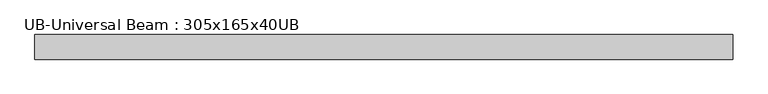
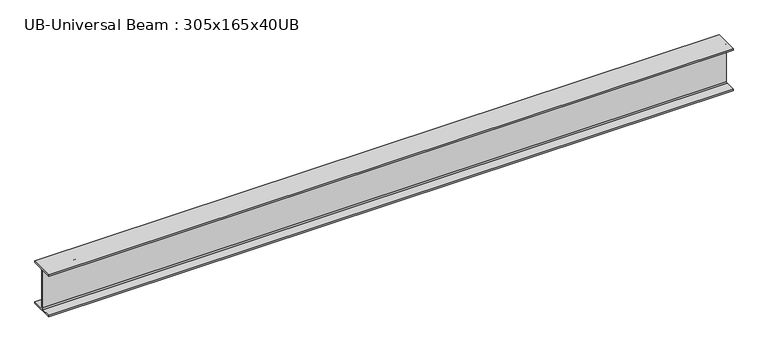
"""IFC4 building model written with IfcOpenShell, lengths in millimetres: beam geometry, UB-Universal Beam : 305x165x40UB."""

from ifc_helpers import new_model, si_unit, point, frame, frame_2d, origin, place, context, project, spatial, polyline, circle_curve, trimmed, segment, composite_curve, outline, extrude, source, transform, mapped, element, save


def ub_universal_beam_305x165x40ub_4e97a9be(model_context):
    return source(origin(), model_context, "Body", "SweptSolid", [
        extrude(outline(composite_curve([segment(polyline([(82.5, -141.5), (82.5, -151.7), (-82.5, -151.7), (-82.5, -141.5), (-11.9, -141.5)]), True, "CONTINUOUS"), segment(trimmed(circle_curve(frame_2d((-11.9, -132.6)), 8.9), [point((-11.9, -141.5))], [point((-3.0, -132.6))], True, "CARTESIAN"), True, "CONTINUOUS"), segment(polyline([(-3.0, -132.6), (-3.0, 132.6)]), True, "CONTINUOUS"), segment(trimmed(circle_curve(frame_2d((-11.9, 132.6)), 8.9), [point((-3.0, 132.6))], [point((-11.9, 141.5))], True, "CARTESIAN"), True, "CONTINUOUS"), segment(polyline([(-11.9, 141.5), (-82.5, 141.5), (-82.5, 151.7), (82.5, 151.7), (82.5, 141.5), (11.9, 141.5)]), True, "CONTINUOUS"), segment(trimmed(circle_curve(frame_2d((11.9, 132.6)), 8.9), [point((11.9, 141.5))], [point((3.0, 132.6))], True, "CARTESIAN"), True, "CONTINUOUS"), segment(polyline([(3.0, 132.6), (3.0, -132.6)]), True, "CONTINUOUS"), segment(trimmed(circle_curve(frame_2d((11.9, -132.6)), 8.9), [point((3.0, -132.6))], [point((11.9, -141.5))], True, "CARTESIAN"), True, "CONTINUOUS"), segment(polyline([(11.9, -141.5), (82.5, -141.5)]), True, "CONTINUOUS")], self_intersect=False)), frame((-2334.65, 0.0, 0.0), z_axis=(1.0, 0.0, 0.0), x_axis=(0.0, 1.0, 0.0)), (0.0, 0.0, 1.0), 4669.3),
    ])


if __name__ == "__main__":
    model = new_model("IFC4")
    model_context = context("Model", 3, world=origin())
    ifc_project = project(units=[si_unit("LENGTHUNIT", "METRE", prefix="MILLI")], contexts=[model_context])
    site = spatial("IfcSite", under=ifc_project)
    building = spatial("IfcBuilding", under=site)
    placement = place(None, origin())
    ub_universal_beam_305x165x40ub_shape = ub_universal_beam_305x165x40ub_4e97a9be(model_context)
    element("IfcBeam", 1, ObjectType="UB-Universal Beam : 305x165x40UB", at=placement, inside=building, context=model_context, shape_type="MappedRepresentation", body=[
        mapped(ub_universal_beam_305x165x40ub_shape, transform((0.0, 0.0, 0.0), x_axis=(1.0, 0.0, 0.0), y_axis=(0.0, 1.0, 0.0), z_axis=(0.0, 0.0, 1.0))),
    ])
    save(model, "model.ifc")

# Revit data of these elements
# Type "UB-Universal Beam : 305x165x40UB"
#   Nominal h = "305"
#   W = 0
#   Start Extension Calculation [instance default] = 3000 mm
#   Start Extension [instance default] = -12.7 mm
#   End Extension Calculation [instance default] = 3000 mm
#   End Extension [instance default] = -12.7 mm
#   Ix = 8503
#   Length [instance default] = 1524 mm
#   M = 40.3
#   Zx = 560
#   b = 165 mm
#   h = 303.4 mm
#   r = 8.9 mm
#   s = 6 mm
#   t = 10.2 mm
#   A = 0.005 m²
#   Structural Material [instance default] = Metal - Steel - 345 MPa
#   Assembly Code = ""
# Element 1 (IfcBeam, "UB-Universal Beam : 305x165x40UB")
#   Materials on its faces: "Metal - Steel - 345 MPa"
# Materials
#   "Metal - Steel - 345 MPa": class "Metal", colour RGB 241 46 46, transparency 0
